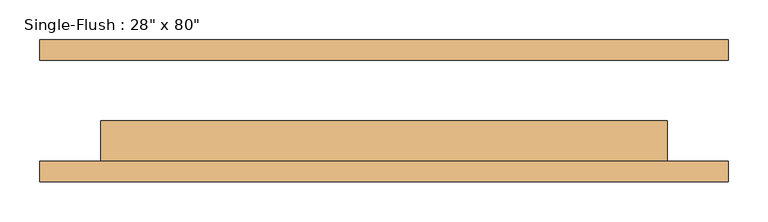
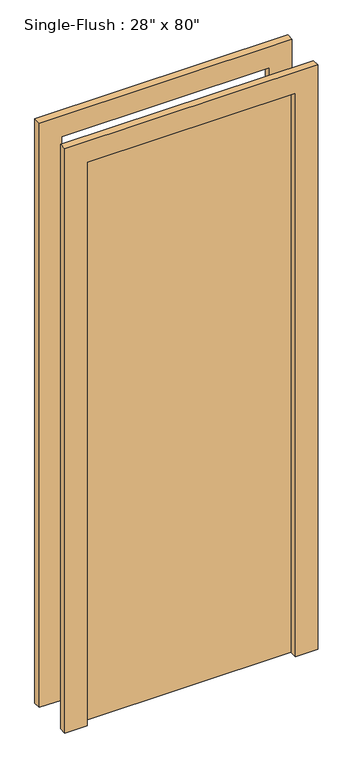
"""IFC4 building model written with IfcOpenShell, lengths in millimetres: door geometry."""

from ifc_helpers import new_model, si_unit, frame, origin, origin_with_axes, place, context, project, spatial, polyline, outline, extrude, source, transform, mapped, element, save


def door_c771f3ba(model_context):
    return source(origin(), model_context, "Body", "SweptSolid", [
        extrude(outline(polyline([(2108.2, -431.8), (0.0, -431.8), (0.0, -355.6), (2032.0, -355.6), (2032.0, 355.6), (0.0, 355.6), (0.0, 431.8), (2108.2, 431.8), (2108.2, -431.8)])), frame((0.0, -88.9, 0.0), z_axis=(0.0, 1.0, 0.0), x_axis=(0.0, 0.0, 1.0)), (0.0, 0.0, 1.0), 25.4),
        extrude(outline(polyline([(2108.2, 431.8), (2108.2, -431.8), (0.0, -431.8), (0.0, -355.6), (2032.0, -355.6), (2032.0, 355.6), (0.0, 355.6), (0.0, 431.8), (2108.2, 431.8)])), frame((0.0, 63.5, 0.0), z_axis=(0.0, 1.0, 0.0), x_axis=(0.0, 0.0, 1.0)), (0.0, 0.0, 1.0), 25.4),
        extrude(outline(polyline([(355.6, -12.7), (355.6, -63.5), (-355.6, -63.5), (-355.6, -12.7), (355.6, -12.7)])), origin_with_axes(), (0.0, 0.0, 1.0), 2032.0),
    ])


if __name__ == "__main__":
    model = new_model("IFC4")
    model_context = context("Model", 3, world=origin())
    ifc_project = project(units=[si_unit("LENGTHUNIT", "METRE", prefix="MILLI")], contexts=[model_context])
    site = spatial("IfcSite", under=ifc_project)
    building = spatial("IfcBuilding", under=site)
    placement = place(None, origin())
    door_shape = door_c771f3ba(model_context)
    element("IfcDoor", 1, ObjectType="Single-Flush : 28\" x 80\"", at=placement, inside=building, context=model_context, shape_type="MappedRepresentation", body=[
        mapped(door_shape, transform((0.0, 0.0, 0.0), x_axis=(1.0, 0.0, 0.0), y_axis=(0.0, 1.0, 0.0), z_axis=(0.0, 0.0, 1.0))),
    ])
    save(model, "model.ifc")

# Revit data of these elements
# Type "Single-Flush : 28\" x 80\""
#   Type Mark = "13"
#   Construction Type Id = "MDOOR"
#   Assembly Code = "C1020"
#   Analytic Construction = "Metal"
#   Thickness = 0' - 2"
#   Heat Transfer Coefficient (U) = 0.651978 BTU/(h·ft²·°F)
#   Height = 6' - 8"
#   Trim Projection Ext = 0' - 1"
#   Trim Projection Int = 0' - 1"
#   Trim Width = 0' - 3"
#   Width = 2' - 4"
#   Define Thermal Properties by = 1
#   Door Material = Door - Panel
#   Frame Material = Door - Frame
#   Visual Light Transmittance = 0
#   Solar Heat Gain Coefficient = 0
#   Function = (empty or 0)
#   Wall Closure = (empty or 0)
# Element 1 (IfcDoor, "Single-Flush : 28\" x 80\"")
#   Materials on its faces: "Door - Frame", "Door - Panel"
# Materials
#   "Door - Panel": class "Wood", colour RGB 210 159 95, transparency 0, Cost = 0
#   "Door - Frame": class "Miscellaneous", colour RGB 118 70 51, transparency 0, Cost = 0
